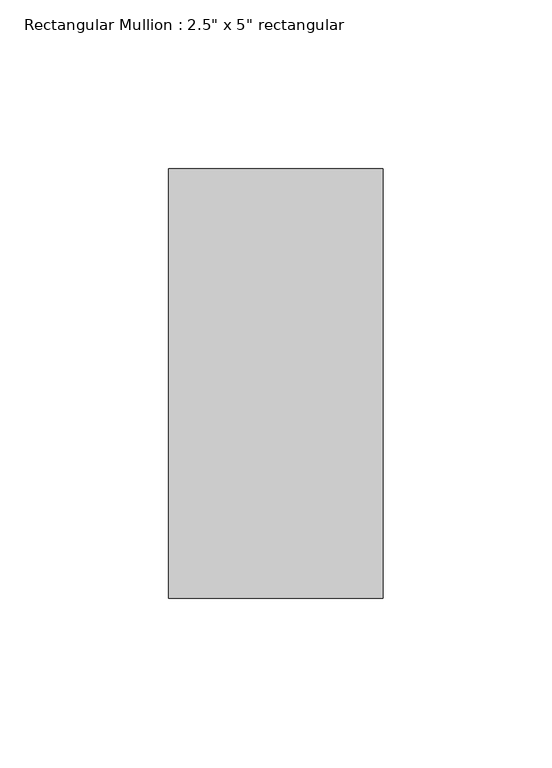
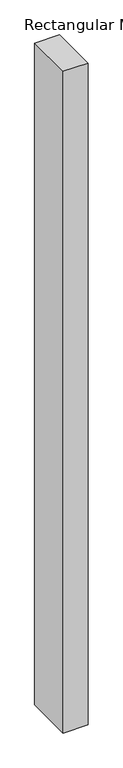
"""IFC4 building model written with IfcOpenShell, lengths in millimetres: member geometry."""

import ifcopenshell
import ifcopenshell.guid

model = None  # the IFC model being written
_history = None  # IfcOwnerHistory: only IFC2X3 demands one
_inside = {}  # id of a spatial element -> (the spatial element, [elements in it])
_under = {}  # id of a project, library or spatial element -> (it, [spatial elements below it])
_declared = {}  # id of a project -> (the project, [libraries it declares])
_typed = {}  # id of a type object -> (the type object, [elements of that type])
_made_of = {}  # id of a material, layer set ... -> (it, [elements and type objects made of it])


def new_model(schema):
    """Start an empty IFC model of exactly this schema.

    Asked for "IFC4X3", IfcOpenShell would pick the latest addendum, in which some entities
    have other attributes; the version numbers below select the first issue.
    IFC2X3 requires an IfcOwnerHistory on every rooted entity: one is made here for all.
    """
    global model, _history
    if schema == "IFC4X3":
        model = ifcopenshell.file(schema_version=(4, 3, 0, 0))
    else:
        model = ifcopenshell.file(schema=schema)
    _inside.clear()
    _under.clear()
    _declared.clear()
    _typed.clear()
    _made_of.clear()
    _history = None
    if model.schema == "IFC2X3":
        org = make("IfcOrganization", Name="unknown")
        user = make(
            "IfcPersonAndOrganization",
            ThePerson=make("IfcPerson", FamilyName="unknown"),
            TheOrganization=org,
        )
        app = make(
            "IfcApplication",
            ApplicationDeveloper=org,
            Version="unknown",
            ApplicationFullName="unknown",
            ApplicationIdentifier="unknown",
        )
        _history = make(
            "IfcOwnerHistory",
            OwningUser=user,
            OwningApplication=app,
            ChangeAction="ADDED",
            CreationDate=0,
        )
    return model


def make(cls, **values):
    """One entity of the class cls with the attributes given. An attribute that is None is left unset."""
    return model.create_entity(
        cls, **{name: value for name, value in values.items() if value is not None}
    )


def rooted(cls, **values):
    """An entity with a GlobalId (a new one), such as an element, a storey or a relation."""
    return make(cls, GlobalId=ifcopenshell.guid.new(), OwnerHistory=_history, **values)


def si_unit(unit_type, name, prefix=None):
    """IfcSIUnit, for example si_unit("LENGTHUNIT", "METRE", prefix="MILLI")."""
    return make("IfcSIUnit", UnitType=unit_type, Prefix=prefix, Name=name)


def assignment(units):
    """IfcUnitAssignment: the units of a project."""
    return None if units is None else make("IfcUnitAssignment", Units=units)


def point(xyz):
    """IfcCartesianPoint."""
    return None if xyz is None else make("IfcCartesianPoint", Coordinates=xyz)


def direction(xyz):
    """IfcDirection."""
    return None if xyz is None else make("IfcDirection", DirectionRatios=xyz)


def frame(location, z_axis=None, x_axis=None):
    """IfcAxis2Placement3D, a coordinate frame: its origin and axes. An axis left out is left unset."""
    return make(
        "IfcAxis2Placement3D",
        Location=point(location),
        Axis=direction(z_axis),
        RefDirection=direction(x_axis),
    )


def origin():
    """The frame at (0, 0, 0) with its axes left unset."""
    return frame((0.0, 0.0, 0.0))


def place(relative_to, where):
    """IfcLocalPlacement: puts the frame where relative to a parent placement (None: the world)."""
    return make(
        "IfcLocalPlacement", PlacementRelTo=relative_to, RelativePlacement=where
    )


def context(
    kind, dimensions, precision=None, world=None, true_north=None, identifier=None
):
    """IfcGeometricRepresentationContext, for example the 3D "Model" context."""
    return make(
        "IfcGeometricRepresentationContext",
        ContextIdentifier=identifier,
        ContextType=kind,
        CoordinateSpaceDimension=dimensions,
        Precision=precision,
        WorldCoordinateSystem=world,
        TrueNorth=true_north,
    )


def project(units=None, contexts=None):
    """IfcProject with its units and contexts."""
    return rooted(
        "IfcProject",
        Name="project",
        RepresentationContexts=contexts,
        UnitsInContext=assignment(units),
    )


def spatial(cls, under=None, at=None, **own):
    """A site, building, storey or space (cls), placed at a placement, below another one or the project."""
    s = rooted(cls, ObjectPlacement=at, **own)
    if under is not None:
        _under.setdefault(under.id(), (under, []))[1].append(s)
    return s


def polyline(points):
    """IfcPolyline through the points."""
    return make("IfcPolyline", Points=[point(p) for p in points])


def outline(outer, holes=None, kind="AREA"):
    """IfcArbitraryClosedProfileDef: a profile drawn as a closed curve; with holes, ...WithVoids."""
    if holes is None:
        return make("IfcArbitraryClosedProfileDef", ProfileType=kind, OuterCurve=outer)
    return make(
        "IfcArbitraryProfileDefWithVoids",
        ProfileType=kind,
        OuterCurve=outer,
        InnerCurves=holes,
    )


def extrude(swept, where, along, depth):
    """IfcExtrudedAreaSolid: the profile swept, set in the frame where, extruded along a direction by depth."""
    return make(
        "IfcExtrudedAreaSolid",
        SweptArea=swept,
        Position=where,
        ExtrudedDirection=direction(along),
        Depth=depth,
    )


def shape(context_of_items, identifier, shape_type, items):
    """IfcShapeRepresentation: the items that make up one representation, for example the "Body"."""
    return make(
        "IfcShapeRepresentation",
        ContextOfItems=context_of_items,
        RepresentationIdentifier=identifier,
        RepresentationType=shape_type,
        Items=items,
    )


def source(mapping_origin, context_of_items, identifier, shape_type, items):
    """IfcRepresentationMap: a shape defined once, which mapped items show again and again."""
    return make(
        "IfcRepresentationMap",
        MappingOrigin=mapping_origin,
        MappedRepresentation=shape(context_of_items, identifier, shape_type, items),
    )


def transform(
    local_origin,
    x_axis=None,
    y_axis=None,
    z_axis=None,
    scale=None,
    scale2=None,
    scale3=None,
    uniform=True,
):
    """IfcCartesianTransformationOperator3D, or its non-uniform kind. x_axis, y_axis, z_axis: its Axis1, 2, 3."""
    if uniform:
        return make(
            "IfcCartesianTransformationOperator3D",
            Axis1=direction(x_axis),
            Axis2=direction(y_axis),
            LocalOrigin=point(local_origin),
            Scale=scale,
            Axis3=direction(z_axis),
        )
    return make(
        "IfcCartesianTransformationOperator3DnonUniform",
        Axis1=direction(x_axis),
        Axis2=direction(y_axis),
        LocalOrigin=point(local_origin),
        Scale=scale,
        Axis3=direction(z_axis),
        Scale2=scale2,
        Scale3=scale3,
    )


def mapped(mapping_source, mapping_target):
    """IfcMappedItem: shows the shape of a source again, moved by a transform."""
    return make(
        "IfcMappedItem", MappingSource=mapping_source, MappingTarget=mapping_target
    )


def made_of(thing, what):
    """Note that an element or type object is made of a material, layer set ...; save() writes the relation."""
    if what is not None:
        _made_of.setdefault(what.id(), (what, []))[1].append(thing)
    return thing


def element(
    cls,
    number,
    at=None,
    inside=None,
    cuts=None,
    type_object=None,
    material=None,
    context=None,
    identifier="Body",
    shape_type=None,
    held_by="IfcProductDefinitionShape",
    body=None,
    shapes=None,
    **own,
):
    """One element of the class cls, such as IfcWall. Its Tag is "e" and its number.

    at: its placement. inside: the storey or other place that contains it. cuts: it is an
    opening in that element (IfcRelVoidsElement). A single representation is given by context,
    identifier, shape_type and body (its items); several are given by shapes. held_by: the class
    of the entity that holds the representations. save() writes the other relations.
    """
    e = rooted(cls, Tag="e%d" % number, ObjectPlacement=at, **own)
    if body is not None:
        shapes = [shape(context, identifier, shape_type, body)]
    if shapes is not None:
        e.Representation = make(held_by, Representations=shapes)
    if inside is not None:
        _inside.setdefault(inside.id(), (inside, []))[1].append(e)
    if cuts is not None:
        rooted(
            "IfcRelVoidsElement", RelatingBuildingElement=cuts, RelatedOpeningElement=e
        )
    if type_object is not None:
        _typed.setdefault(type_object.id(), (type_object, []))[1].append(e)
    return made_of(e, material)


def aggregate(whole, parts):
    """IfcRelAggregates: a whole, such as a stair, and the parts it consists of."""
    return rooted("IfcRelAggregates", RelatingObject=whole, RelatedObjects=parts)


def save(model, path):
    """Write the relations noted so far, then the file.

    IfcRelAggregates (storeys below a building ...), IfcRelContainedInSpatialStructure (elements
    in a storey), IfcRelDefinesByType, IfcRelAssociatesMaterial and IfcRelDeclares: one each for
    every whole, place, type object, material and project.
    """
    for whole, parts in _under.values():
        aggregate(whole, parts)
    for where, things in _inside.values():
        rooted(
            "IfcRelContainedInSpatialStructure",
            RelatedElements=things,
            RelatingStructure=where,
        )
    for kind, things in _typed.values():
        rooted("IfcRelDefinesByType", RelatedObjects=things, RelatingType=kind)
    for what, things in _made_of.values():
        rooted("IfcRelAssociatesMaterial", RelatedObjects=things, RelatingMaterial=what)
    for by, libraries in _declared.values():
        rooted("IfcRelDeclares", RelatingContext=by, RelatedDefinitions=libraries)
    model.write(path)


def member_c3fe432b(model_context):
    return source(origin(), model_context, "Body", "SweptSolid", [
        extrude(outline(polyline([(31.75, 63.5), (31.75, -63.5), (-31.75, -63.5), (-31.75, 63.5), (31.75, 63.5)])), frame((0.0, 0.0, -1797.05), z_axis=(0.0, 0.0, 1.0), x_axis=(1.0, 0.0, 0.0)), (0.0, 0.0, 1.0), 1797.05),
    ])


if __name__ == "__main__":
    model = new_model("IFC4")
    model_context = context("Model", 3, world=origin())
    ifc_project = project(units=[si_unit("LENGTHUNIT", "METRE", prefix="MILLI")], contexts=[model_context])
    site = spatial("IfcSite", under=ifc_project)
    building = spatial("IfcBuilding", under=site)
    placement = place(None, origin())
    member_shape = member_c3fe432b(model_context)
    element("IfcMember", 1, ObjectType="Rectangular Mullion : 2.5\" x 5\" rectangular", at=placement, inside=building, context=model_context, shape_type="MappedRepresentation", body=[
        mapped(member_shape, transform((0.0, 0.0, 0.0), x_axis=(1.0, 0.0, 0.0), y_axis=(0.0, 1.0, 0.0), z_axis=(0.0, 0.0, 1.0))),
    ])
    save(model, "model.ifc")

# Revit data of these elements
# Type "Rectangular Mullion : 2.5\" x 5\" rectangular"
#   built-in parameter 1007304 = 0.416667 (stored number, unit not read)
#   built-in parameter 1007301 = 0.104167 (stored number, unit not read)
#   built-in parameter 1007300 = 0.104167 (stored number, unit not read)
# Element 1 (IfcMember, "Rectangular Mullion : 2.5\" x 5\" rectangular")
#   Materials on its faces: "Aluminum"
# Materials
#   "Aluminum": class "Metal", colour RGB 247 247 247, transparency 0, Description = "Aluminum 6061", Cost = 0
